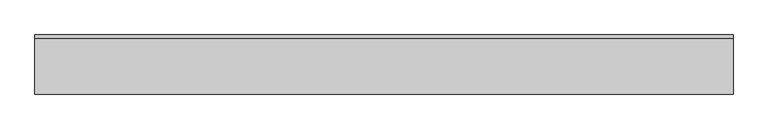
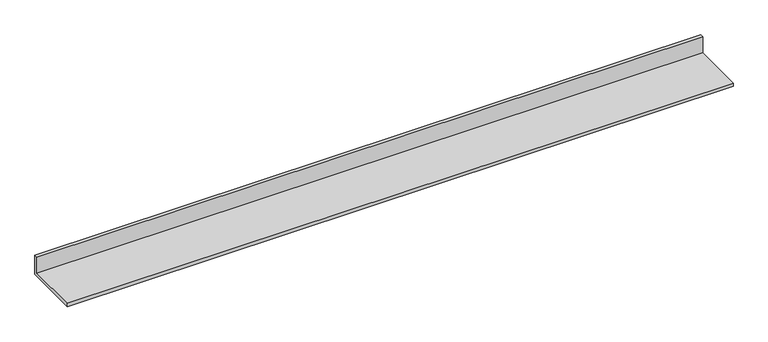
"""IFC4 building model written with IfcOpenShell, lengths in millimetres: proxy geometry, 거터3 : 거터2."""

from ifc_helpers import new_model, si_unit, frame, origin, place, context, project, spatial, polyline, outline, extrude, source, transform, mapped, element, save


def generic_models_a722396c(model_context):
    return source(origin(), model_context, "Body", "SweptSolid", [
        extrude(outline(polyline([(20999.5208589, 6299.9720055), (20159.5208589, 6299.9720055), (20159.5208589, 6349.9720055), (20949.5208589, 6349.9720055), (20949.5208589, 6599.2986846), (20999.5208589, 6599.2986846), (20999.5208589, 6299.9720055)])), frame((40675.0, 0.0, 0.0), z_axis=(1.0, 0.0, 0.0), x_axis=(0.0, 1.0, 0.0)), (0.0, 0.0, 1.0), 9925.0),
    ])


if __name__ == "__main__":
    model = new_model("IFC4")
    model_context = context("Model", 3, world=origin())
    ifc_project = project(units=[si_unit("LENGTHUNIT", "METRE", prefix="MILLI")], contexts=[model_context])
    site = spatial("IfcSite", under=ifc_project)
    building = spatial("IfcBuilding", under=site)
    placement = place(None, origin())
    generic_models_shape = generic_models_a722396c(model_context)
    element("IfcBuildingElementProxy", 1, Name="거터3 : 거터2", ObjectType="거터3 : 거터2", at=placement, inside=building, context=model_context, shape_type="MappedRepresentation", body=[
        mapped(generic_models_shape, transform((0.0, 0.0, 0.0), x_axis=(1.0, 0.0, 0.0), y_axis=(0.0, 1.0, 0.0), z_axis=(0.0, 0.0, 1.0))),
    ])
    save(model, "model.ifc")
